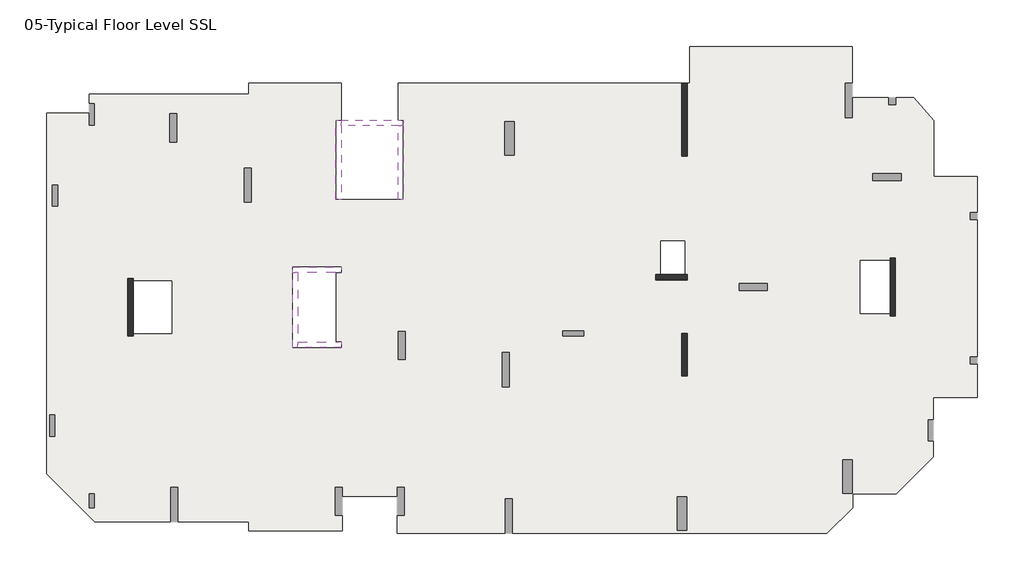
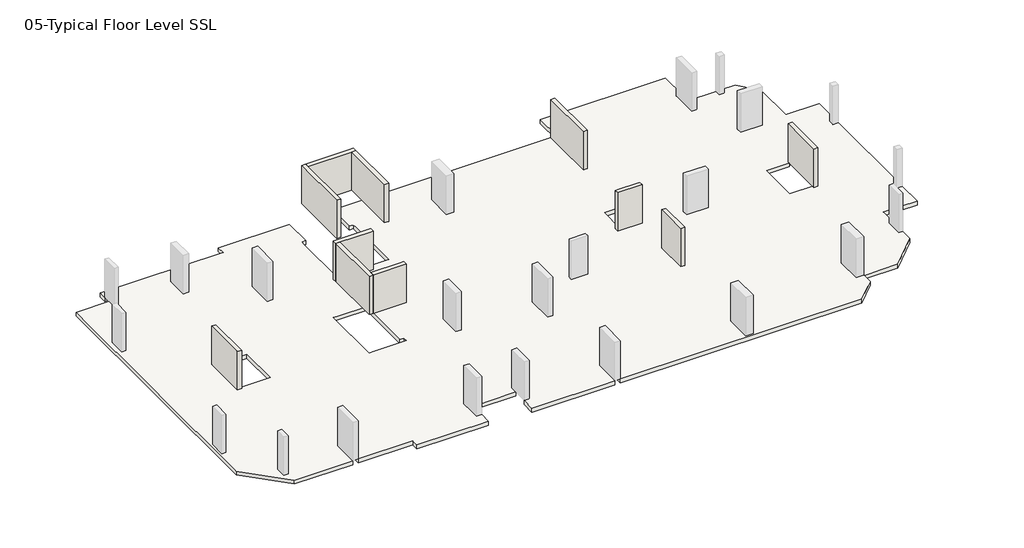
# One storey, part 1 of 2: 11 walls, 1 slab.
"""IFC4 building model written with IfcOpenShell, lengths in millimetres."""

from ifc_helpers import new_model, si_unit, origin, place, context, project, spatial, faceted_brep, element, save

model = new_model("IFC4")

# Units and contexts
model_context = context("Model", 3, world=origin())
ifc_project = project(units=[si_unit("LENGTHUNIT", "METRE", prefix="MILLI")], contexts=[model_context])

# Site, building, storey
site = spatial("IfcSite", under=ifc_project)
building = spatial("IfcBuilding", under=site)
storey = spatial("IfcBuildingStorey", under=building, Name="05-Typical Floor Level SSL", Elevation=9000.0)

# Slab
placement = place(None, origin())
element("IfcSlab", 1, ObjectType="Generic 300mm", at=placement, inside=storey, context=model_context, shape_type="Brep", body=[
    faceted_brep([(36192.0021644, 24072.000519, 8700.0), (36192.0021644, 26172.000519, 8700.0), (45446.0007483, 26172.000519, 8700.0), (45446.0007483, 24087.0, 8700.0), (45046.0007483, 24087.0, 8700.0), (45046.0007483, 22137.0, 8700.0), (45446.0007483, 22137.0, 8700.0), (45446.0007483, 23252.0000315, 8700.0), (47498.6337868, 23252.0000315, 8700.0), (47498.6337868, 22852.0, 8700.0), (47898.6337868, 22852.0, 8700.0), (47898.6337868, 23252.0000315, 8700.0), (48936.764334, 23252.0000315, 8700.0), (50076.0016214, 21956.8283806, 8700.0), (50076.0016214, 18780.0084406, 8700.0), (52549.9999998, 18780.0084406, 8700.0), (52549.9999998, 16712.0, 8700.0), (52149.9999998, 16712.0, 8700.0), (52149.9999998, 16312.0, 8700.0), (52549.9999998, 16312.0, 8700.0), (52549.9999998, 8504.0039609, 8700.0), (52149.9999998, 8504.0039609, 8700.0), (52149.9999998, 8104.0039609, 8700.0), (52549.9999998, 8104.0039609, 8700.0), (52549.9999998, 6204.0084406, 8700.0), (50046.0009271, 6204.0084406, 8700.0), (50046.0009271, 4931.9999929, 8700.0), (49746.0009271, 4931.9999929, 8700.0), (49746.0009271, 3731.9999929, 8700.0), (50046.0009271, 3731.9999929, 8700.0), (50046.0009271, 2810.5958657, 8700.0), (47943.4055804, 708.000519, 8700.0), (45456.0017287, 708.000519, 8700.0), (45456.0017287, -61.7051085, 8700.0), (43990.7023722, -1527.004465, 8700.0), (26113.9999998, -1527.004465, 8700.0), (26113.9999998, 422.995535, 8700.0), (25713.9999998, 422.995535, 8700.0), (25713.9999998, -1527.004465, 8700.0), (19569.9997488, -1527.004465, 8700.0), (19569.9997488, -512.0044652, 8700.0), (19969.9997488, -512.0044652, 8700.0), (19969.9997488, 1087.9955348, 8700.0), (19569.9997488, 1087.9955348, 8700.0), (19569.9997488, 564.000519, 8700.0), (16429.9999981, 564.000519, 8700.0), (16429.9999981, 1088.0, 8700.0), (16029.9999981, 1088.0, 8700.0), (16029.9999981, -512.0, 8700.0), (16429.9999981, -512.0, 8700.0), (16429.9999981, -1391.999481, 8700.0), (11136.0000923, -1391.999481, 8700.0), (11136.0000923, -866.9999847, 8700.0), (7082.0000416, -866.9999847, 8700.0), (7082.0000416, 1083.0000153, 8700.0), (6682.0000416, 1083.0000153, 8700.0), (6682.0000416, -866.9999847, 8700.0), (2364.4419097, -866.9999847, 8700.0), (-372.0, 1869.441925, 8700.0), (-372.0, 22380.0004589, 8700.0), (2052.0, 22380.0004589, 8700.0), (2052.0, 21708.0000656, 8700.0), (2352.0, 21708.0000656, 8700.0), (2352.0, 22908.0000656, 8700.0), (2052.0, 22908.0000656, 8700.0), (2052.0, 23472.000519, 8700.0), (11136.0000923, 23472.000519, 8700.0), (11136.0000923, 24072.000519, 8700.0), (16380.0000168, 24072.000519, 8700.0), (16380.0000168, 21972.0, 8700.0), (16079.9999997, 21972.0, 8700.0), (16079.9999997, 21672.0, 8700.0), (16079.9999997, 17468.0, 8700.0), (16379.9999997, 17468.0, 8700.0), (19619.9999997, 17468.0, 8700.0), (19919.9999997, 17468.0, 8700.0), (19919.9999997, 21672.0, 8700.0), (19919.9999997, 21972.0, 8700.0), (19619.9997365, 21972.0, 8700.0), (19619.9997365, 24072.000519, 8700.0), (35747.9999998, 24072.000519, 8700.0), (35747.9999998, 19932.0, 8700.0), (36047.9999998, 19932.0, 8700.0), (36047.9999998, 24072.000519, 8700.0), (16079.9999907, 9359.999998, 8700.0), (16079.9999907, 13320.0000002, 8700.0), (16380.0000168, 13320.0000002, 8700.0), (16380.0000168, 13620.0000002, 8700.0), (13919.9999907, 13620.0000002, 8700.0), (13619.9999907, 13620.0000002, 8700.0), (13619.9999907, 13320.0000002, 8700.0), (13619.9999907, 9359.999998, 8700.0), (13619.9999907, 9059.999998, 8700.0), (13919.9999907, 9059.999998, 8700.0), (16380.0000168, 9059.999998, 8700.0), (16380.0000168, 9359.999998, 8700.0), (257.9999999, 17088.0, 8700.0), (257.9999999, 18288.0, 8700.0), (-42.0000001, 18288.0, 8700.0), (-42.0000001, 17088.0, 8700.0), (108.001803, 4001.9999858, 8700.0), (108.001803, 5201.9999858, 8700.0), (-191.998197, 5201.9999858, 8700.0), (-191.998197, 4001.9999858, 8700.0), (30175.9999998, 9996.0000019, 8700.0), (28975.9999998, 9996.0000019, 8700.0), (28975.9999998, 9696.0000019, 8700.0), (30175.9999998, 9696.0000019, 8700.0), (7021.9999999, 20740.0000078, 8700.0), (7021.9999999, 22340.0000078, 8700.0), (6621.9999999, 22340.0000078, 8700.0), (6621.9999999, 20740.0000078, 8700.0), (48205.9993605, 18950.0, 8700.0), (46605.9993605, 18950.0, 8700.0), (46605.9993605, 18550.0, 8700.0), (48205.9993605, 18550.0, 8700.0), (20030.000009, 8355.9999979, 8700.0), (20030.000009, 9955.9999979, 8700.0), (19630.000009, 9955.9999979, 8700.0), (19630.000009, 8355.9999979, 8700.0), (11270.0000427, 17312.9999996, 8700.0), (11270.0000427, 19262.9999996, 8700.0), (10870.0000427, 19262.9999996, 8700.0), (10870.0000427, 17312.9999996, 8700.0), (40598.0014887, 12692.0079212, 8700.0), (38998.0014887, 12692.0079212, 8700.0), (38998.0014887, 12292.0079212, 8700.0), (40598.0014887, 12292.0079212, 8700.0), (25934.0000455, 6801.0001824, 8700.0), (25934.0000455, 8751.0001824, 8700.0), (25534.0000455, 8751.0001824, 8700.0), (25534.0000455, 6801.0001824, 8700.0), (36035.9999998, -1351.9992017, 8700.0), (36035.9999998, 548.0007983, 8700.0), (35485.9999998, 548.0007983, 8700.0), (35485.9999998, -1351.9992017, 8700.0), (45443.9999998, 748.0, 8700.0), (45443.9999998, 2648.0, 8700.0), (44893.9999998, 2648.0, 8700.0), (44893.9999998, 748.0, 8700.0), (26218.9999998, 20000.0, 8700.0), (26218.9999998, 21900.0, 8700.0), (25668.9999998, 21900.0, 8700.0), (25668.9999998, 20000.0, 8700.0), (2352.0, -72.0, 8700.0), (2352.0, 728.0, 8700.0), (2052.0, 728.0, 8700.0), (2052.0, -72.0, 8700.0), (4248.0000025, 12984.0000001, 8700.0), (4248.0000025, 9696.0, 8700.0), (4548.0000025, 9696.0, 8700.0), (4548.0000025, 9840.0000003, 8700.0), (6743.9999995, 9840.0000003, 8700.0), (6743.9999995, 12840.0000003, 8700.0), (4548.0000034, 12840.0000003, 8700.0), (4548.0000025, 12984.0000001, 8700.0), (34248.0015201, 12899.9999992, 8700.0), (36048.0015201, 12899.9999992, 8700.0), (36048.0015201, 13199.9999992, 8700.0), (35904.002157, 13199.9999992, 8700.0), (35904.002157, 15108.0000083, 8700.0), (34548.0015145, 15108.0000083, 8700.0), (34548.0015145, 13199.9999992, 8700.0), (34248.0015201, 13199.9999992, 8700.0), (35748.0054035, 9840.0000002, 8700.0), (35748.0054035, 7428.0000762, 8700.0), (36048.0054035, 7428.0000762, 8700.0), (36048.0054035, 9840.0000002, 8700.0), (47580.0014811, 14136.0000002, 8700.0), (47580.0014811, 13992.0079177, 8700.0), (45900.001729, 13992.0079177, 8700.0), (45900.001729, 10992.0079181, 8700.0), (47580.0014798, 10992.0079181, 8700.0), (47580.0014811, 10848.0079202, 8700.0), (47880.0014811, 10848.0079202, 8700.0), (47880.0014811, 14136.0000002, 8700.0), (36192.0021644, 26172.000519, 9000.0), (36192.0021644, 24072.000519, 9000.0), (36047.9999998, 24072.000519, 9000.0), (36047.9999998, 19932.0, 9000.0), (35747.9999998, 19932.0, 9000.0), (35747.9999998, 24072.000519, 9000.0), (19619.9997365, 24072.000519, 9000.0), (19619.9997365, 21972.0, 9000.0), (19919.9999997, 21972.0, 9000.0), (19919.9999997, 21672.0, 9000.0), (19919.9999997, 17468.0, 9000.0), (19619.9999997, 17468.0, 9000.0), (16379.9999997, 17468.0, 9000.0), (16079.9999997, 17468.0, 9000.0), (16079.9999997, 21672.0, 9000.0), (16079.9999997, 21972.0, 9000.0), (16380.0000168, 21972.0, 9000.0), (16380.0000168, 24072.000519, 9000.0), (11136.0000923, 24072.000519, 9000.0), (11136.0000923, 23472.000519, 9000.0), (2052.0, 23472.000519, 9000.0), (2052.0, 22908.0000656, 9000.0), (2352.0, 22908.0000656, 9000.0), (2352.0, 21708.0000656, 9000.0), (2052.0, 21708.0000656, 9000.0), (2052.0, 22380.0004589, 9000.0), (-372.0, 22380.0004589, 9000.0), (-372.0, 1869.441925, 9000.0), (2364.4419097, -866.9999847, 9000.0), (6682.0000416, -866.9999847, 9000.0), (6682.0000416, 1083.0000153, 9000.0), (7082.0000416, 1083.0000153, 9000.0), (7082.0000416, -866.9999847, 9000.0), (11136.0000923, -866.9999847, 9000.0), (11136.0000923, -1391.999481, 9000.0), (16429.9999981, -1391.999481, 9000.0), (16429.9999981, -512.0, 9000.0), (16029.9999981, -512.0, 9000.0), (16029.9999981, 1088.0, 9000.0), (16429.9999981, 1088.0, 9000.0), (16429.9999981, 564.000519, 9000.0), (19569.9997488, 564.000519, 9000.0), (19569.9997488, 1087.9955348, 9000.0), (19969.9997488, 1087.9955348, 9000.0), (19969.9997488, -512.0044652, 9000.0), (19569.9997488, -512.0044652, 9000.0), (19569.9997488, -1527.004465, 9000.0), (25713.9999998, -1527.004465, 9000.0), (25713.9999998, 422.995535, 9000.0), (26113.9999998, 422.995535, 9000.0), (26113.9999998, -1527.004465, 9000.0), (43990.7023722, -1527.004465, 9000.0), (45456.0017287, -61.7051085, 9000.0), (45456.0017287, 708.000519, 9000.0), (47943.4055804, 708.000519, 9000.0), (50046.0009271, 2810.5958657, 9000.0), (50046.0009271, 3731.9999929, 9000.0), (49746.0009271, 3731.9999929, 9000.0), (49746.0009271, 4931.9999929, 9000.0), (50046.0009271, 4931.9999929, 9000.0), (50046.0009271, 6204.0084406, 9000.0), (52549.9999998, 6204.0084406, 9000.0), (52549.9999998, 8104.0039609, 9000.0), (52149.9999998, 8104.0039609, 9000.0), (52149.9999998, 8504.0039609, 9000.0), (52549.9999998, 8504.0039609, 9000.0), (52549.9999998, 16312.0, 9000.0), (52149.9999998, 16312.0, 9000.0), (52149.9999998, 16712.0, 9000.0), (52549.9999998, 16712.0, 9000.0), (52549.9999998, 18780.0084406, 9000.0), (50076.0016214, 18780.0084406, 9000.0), (50076.0016214, 21956.8283806, 9000.0), (48936.764334, 23252.0000315, 9000.0), (47898.6337868, 23252.0000315, 9000.0), (47898.6337868, 22852.0, 9000.0), (47498.6337868, 22852.0, 9000.0), (47498.6337868, 23252.0000315, 9000.0), (45446.0006898, 23252.0000315, 9000.0), (45446.0007483, 22137.0, 9000.0), (45046.0007483, 22137.0, 9000.0), (45046.0007483, 24087.0, 9000.0), (45446.0007483, 24087.0, 9000.0), (45446.0007483, 26172.000519, 9000.0), (16079.9999907, 13320.0000002, 9000.0), (16079.9999907, 9359.999998, 9000.0), (16380.0000168, 9359.999998, 9000.0), (16380.0000168, 9059.999998, 9000.0), (13919.9999907, 9059.999998, 9000.0), (13619.9999907, 9059.999998, 9000.0), (13619.9999907, 9359.999998, 9000.0), (13619.9999907, 13320.0000002, 9000.0), (13619.9999907, 13620.0000002, 9000.0), (13919.9999907, 13620.0000002, 9000.0), (16380.0000168, 13620.0000002, 9000.0), (16380.0000168, 13320.0000002, 9000.0), (257.9999999, 18288.0, 9000.0), (257.9999999, 17088.0, 9000.0), (-42.0000001, 17088.0, 9000.0), (-42.0000001, 18288.0, 9000.0), (108.001803, 5201.9999858, 9000.0), (108.001803, 4001.9999858, 9000.0), (-191.998197, 4001.9999858, 9000.0), (-191.998197, 5201.9999858, 9000.0), (28975.9999998, 9996.0000019, 9000.0), (30175.9999998, 9996.0000019, 9000.0), (30175.9999998, 9696.0000019, 9000.0), (28975.9999998, 9696.0000019, 9000.0), (7021.9999999, 22340.0000078, 9000.0), (7021.9999999, 20740.0000078, 9000.0), (6621.9999999, 20740.0000078, 9000.0), (6621.9999999, 22340.0000078, 9000.0), (46605.9993605, 18950.0, 9000.0), (48205.9993605, 18950.0, 9000.0), (48205.9993605, 18550.0, 9000.0), (46605.9993605, 18550.0, 9000.0), (20030.000009, 9955.9999979, 9000.0), (20030.000009, 8355.9999979, 9000.0), (19630.000009, 8355.9999979, 9000.0), (19630.000009, 9955.9999979, 9000.0), (11270.0000427, 19262.9999996, 9000.0), (11270.0000427, 17312.9999996, 9000.0), (10870.0000427, 17312.9999996, 9000.0), (10870.0000427, 19262.9999996, 9000.0), (38998.0014887, 12692.0079212, 9000.0), (40598.0014887, 12692.0079212, 9000.0), (40598.0014887, 12292.0079212, 9000.0), (38998.0014887, 12292.0079212, 9000.0), (25934.0000455, 8751.0001824, 9000.0), (25934.0000455, 6801.0001824, 9000.0), (25534.0000455, 6801.0001824, 9000.0), (25534.0000455, 8751.0001824, 9000.0), (36035.9999998, 548.0007983, 9000.0), (36035.9999998, -1351.9992017, 9000.0), (35485.9999998, -1351.9992017, 9000.0), (35485.9999998, 548.0007983, 9000.0), (45443.9999998, 2648.0, 9000.0), (45443.9999998, 748.0, 9000.0), (44893.9999998, 748.0, 9000.0), (44893.9999998, 2648.0, 9000.0), (26218.9999998, 21900.0, 9000.0), (26218.9999998, 20000.0, 9000.0), (25668.9999998, 20000.0, 9000.0), (25668.9999998, 21900.0, 9000.0), (4248.0000025, 9696.0, 9000.0), (4248.0000025, 12984.0000001, 9000.0), (4548.0000025, 12984.0000001, 9000.0), (4548.0000025, 12840.0000003, 9000.0), (6743.9999995, 12840.0000003, 9000.0), (6743.9999995, 9840.0000003, 9000.0), (4548.0000034, 9840.0000003, 9000.0), (4548.0000025, 9696.0, 9000.0), (36048.0015201, 12899.9999992, 9000.0), (34248.0015201, 12899.9999992, 9000.0), (34248.0015201, 13199.9999992, 9000.0), (34548.0015145, 13199.9999992, 9000.0), (34548.0015145, 15108.0000083, 9000.0), (35904.002157, 15108.0000083, 9000.0), (35904.002157, 13199.9999992, 9000.0), (36048.0015201, 13199.9999992, 9000.0), (35748.0054035, 7428.0000762, 9000.0), (35748.0054035, 9840.0000002, 9000.0), (36048.0054035, 9840.0000002, 9000.0), (36048.0054035, 7428.0000762, 9000.0), (47880.0014811, 14136.0000002, 9000.0), (47880.0014811, 10848.0079202, 9000.0), (47580.0014811, 10848.0079202, 9000.0), (47580.0014811, 10992.0079181, 9000.0), (45900.001729, 10992.0079181, 9000.0), (45900.001729, 13992.0079177, 9000.0), (47580.0014798, 13992.0079177, 9000.0), (47580.0014811, 14136.0000002, 9000.0), (2352.0, 728.0, 9000.0), (2352.0, -72.0, 9000.0), (2052.0, -72.0, 9000.0), (2052.0, 728.0, 9000.0)], [[[0, 1, 2, 3, 4, 5, 6, 7, 8, 9, 10, 11, 12, 13, 14, 15, 16, 17, 18, 19, 20, 21, 22, 23, 24, 25, 26, 27, 28, 29, 30, 31, 32, 33, 34, 35, 36, 37, 38, 39, 40, 41, 42, 43, 44, 45, 46, 47, 48, 49, 50, 51, 52, 53, 54, 55, 56, 57, 58, 59, 60, 61, 62, 63, 64, 65, 66, 67, 68, 69, 70, 71, 72, 73, 74, 75, 76, 77, 78, 79, 80, 81, 82, 83], [84, 85, 86, 87, 88, 89, 90, 91, 92, 93, 94, 95], [96, 97, 98, 99], [100, 101, 102, 103], [104, 105, 106, 107], [108, 109, 110, 111], [112, 113, 114, 115], [116, 117, 118, 119], [120, 121, 122, 123], [124, 125, 126, 127], [128, 129, 130, 131], [132, 133, 134, 135], [136, 137, 138, 139], [140, 141, 142, 143], [144, 145, 146, 147], [148, 149, 150, 151, 152, 153, 154, 155], [156, 157, 158, 159, 160, 161, 162, 163], [164, 165, 166, 167], [168, 169, 170, 171, 172, 173, 174, 175]], [[176, 177, 178, 179, 180, 181, 182, 183, 184, 185, 186, 187, 188, 189, 190, 191, 192, 193, 194, 195, 196, 197, 198, 199, 200, 201, 202, 203, 204, 205, 206, 207, 208, 209, 210, 211, 212, 213, 214, 215, 216, 217, 218, 219, 220, 221, 222, 223, 224, 225, 226, 227, 228, 229, 230, 231, 232, 233, 234, 235, 236, 237, 238, 239, 240, 241, 242, 243, 244, 245, 246, 247, 248, 249, 250, 251, 252, 253, 254, 255, 256, 257, 258, 259], [260, 261, 262, 263, 264, 265, 266, 267, 268, 269, 270, 271], [272, 273, 274, 275], [276, 277, 278, 279], [280, 281, 282, 283], [284, 285, 286, 287], [288, 289, 290, 291], [292, 293, 294, 295], [296, 297, 298, 299], [300, 301, 302, 303], [304, 305, 306, 307], [308, 309, 310, 311], [312, 313, 314, 315], [316, 317, 318, 319], [320, 321, 322, 323, 324, 325, 326, 327], [328, 329, 330, 331, 332, 333, 334, 335], [336, 337, 338, 339], [340, 341, 342, 343, 344, 345, 346, 347], [348, 349, 350, 351]], [[68, 193, 192, 69]], [[182, 79, 78, 183]], [[79, 182, 181, 80]], [[177, 0, 83, 178]], [[1, 0, 177, 176]], [[2, 1, 176, 259]], [[3, 2, 259, 258]], [[249, 12, 11, 250]], [[7, 254, 253, 8]], [[13, 12, 249, 248]], [[14, 13, 248, 247]], [[15, 14, 247, 246]], [[15, 246, 245, 16]], [[237, 24, 23, 238]], [[19, 242, 241, 20]], [[25, 24, 237, 236]], [[25, 236, 235, 26]], [[30, 29, 232, 231]], [[32, 31, 230, 229]], [[33, 32, 229, 228]], [[34, 33, 228, 227]], [[34, 227, 226, 35]], [[222, 39, 38, 223]], [[39, 222, 221, 40]], [[45, 44, 217, 216]], [[211, 50, 49, 212]], [[51, 50, 211, 210]], [[52, 51, 210, 209]], [[52, 209, 208, 53]], [[204, 57, 56, 205]], [[58, 57, 204, 203]], [[59, 58, 203, 202]], [[60, 59, 202, 201]], [[196, 65, 64, 197]], [[66, 65, 196, 195]], [[67, 66, 195, 194]], [[68, 67, 194, 193]], [[85, 84, 261, 260]], [[62, 199, 198, 63]], [[199, 62, 61, 200]], [[200, 61, 60, 201]], [[63, 198, 197, 64]], [[96, 273, 272, 97]], [[273, 96, 99, 274]], [[274, 99, 98, 275]], [[275, 98, 97, 272]], [[100, 277, 276, 101]], [[277, 100, 103, 278]], [[278, 103, 102, 279]], [[279, 102, 101, 276]], [[28, 233, 232, 29]], [[233, 28, 27, 234]], [[234, 27, 26, 235]], [[104, 281, 280, 105]], [[281, 104, 107, 282]], [[282, 107, 106, 283]], [[283, 106, 105, 280]], [[108, 285, 284, 109]], [[285, 108, 111, 286]], [[286, 111, 110, 287]], [[287, 110, 109, 284]], [[41, 220, 219, 42]], [[220, 41, 40, 221]], [[43, 218, 217, 44]], [[218, 43, 42, 219]], [[112, 289, 288, 113]], [[289, 112, 115, 290]], [[290, 115, 114, 291]], [[291, 114, 113, 288]], [[116, 293, 292, 117]], [[293, 116, 119, 294]], [[294, 119, 118, 295]], [[295, 118, 117, 292]], [[215, 46, 45, 216]], [[48, 213, 212, 49]], [[213, 48, 47, 214]], [[214, 47, 46, 215]], [[120, 297, 296, 121]], [[297, 120, 123, 298]], [[298, 123, 122, 299]], [[299, 122, 121, 296]], [[207, 54, 53, 208]], [[55, 206, 205, 56]], [[206, 55, 54, 207]], [[225, 36, 35, 226]], [[37, 224, 223, 38]], [[224, 37, 36, 225]], [[6, 255, 254, 7]], [[255, 6, 5, 256]], [[256, 5, 4, 257]], [[257, 4, 3, 258]], [[124, 301, 300, 125]], [[301, 124, 127, 302]], [[302, 127, 126, 303]], [[303, 126, 125, 300]], [[128, 305, 304, 129]], [[305, 128, 131, 306]], [[306, 131, 130, 307]], [[307, 130, 129, 304]], [[132, 309, 308, 133]], [[309, 132, 135, 310]], [[310, 135, 134, 311]], [[311, 134, 133, 308]], [[136, 313, 312, 137]], [[313, 136, 139, 314]], [[314, 139, 138, 315]], [[315, 138, 137, 312]], [[140, 317, 316, 141]], [[317, 140, 143, 318]], [[318, 143, 142, 319]], [[319, 142, 141, 316]], [[144, 349, 348, 145]], [[349, 144, 147, 350]], [[146, 351, 350, 147]], [[145, 348, 351, 146]], [[70, 191, 190, 189, 72, 71]], [[191, 70, 69, 192]], [[77, 184, 183, 78]], [[184, 77, 76, 75, 186, 185]], [[271, 86, 85, 260]], [[87, 270, 269, 268, 89, 88]], [[86, 271, 270, 87]], [[89, 268, 267, 266, 265, 92, 91, 90]], [[92, 265, 264, 263, 94, 93]], [[95, 262, 261, 84]], [[262, 95, 94, 263]], [[322, 155, 154, 323]], [[150, 327, 326, 151]], [[148, 321, 320, 149]], [[155, 322, 321, 148]], [[327, 150, 149, 320]], [[156, 329, 328, 157]], [[158, 335, 334, 159]], [[330, 163, 162, 331]], [[157, 328, 335, 158]], [[329, 156, 163, 330]], [[164, 337, 336, 165]], [[166, 339, 338, 167]], [[165, 336, 339, 166]], [[337, 164, 167, 338]], [[342, 173, 172, 343]], [[168, 347, 346, 169]], [[174, 341, 340, 175]], [[173, 342, 341, 174]], [[347, 168, 175, 340]], [[82, 179, 178, 83]], [[180, 81, 80, 181]], [[179, 82, 81, 180]], [[72, 189, 188, 187, 186, 75, 74, 73]], [[325, 152, 151, 326]], [[152, 325, 324, 153]], [[153, 324, 323, 154]], [[345, 170, 169, 346]], [[170, 345, 344, 171]], [[171, 344, 343, 172]], [[160, 333, 332, 161]], [[161, 332, 331, 162]], [[333, 160, 159, 334]], [[31, 30, 231, 230]], [[18, 243, 242, 19]], [[243, 18, 17, 244]], [[244, 17, 16, 245]], [[10, 251, 250, 11]], [[251, 10, 9, 252]], [[252, 9, 8, 253]], [[22, 239, 238, 23]], [[239, 22, 21, 240]], [[240, 21, 20, 241]]]),
])

# Walls
element("IfcWall", 2, ObjectType="Shear Walls 300mm", at=placement, inside=storey, context=model_context, shape_type="Brep", body=[
    faceted_brep([(4548.0000025, 9696.0, 9000.0), (4548.0000025, 12984.0000001, 9000.0), (4548.0000025, 12984.0000001, 11700.0), (4548.0000025, 12984.0000001, 12000.0), (4548.0000025, 12840.0000003, 12000.0), (4548.0000025, 9840.0000003, 12000.0), (4548.0000025, 9696.0, 12000.0), (4548.0000025, 9696.0, 11700.0), (4248.0000025, 9696.0, 9000.0), (4248.0000025, 9696.0, 11700.0), (4248.0000025, 9696.0, 12000.0), (4248.0000025, 12984.0000001, 12000.0), (4248.0000025, 12984.0000001, 11700.0), (4248.0000025, 12984.0000001, 9000.0)], [[[0, 1, 2, 3, 4, 5, 6, 7]], [[8, 9, 10, 11, 12, 13]], [[1, 0, 8, 13]], [[3, 2, 1, 13, 12, 11]], [[6, 5, 4, 3, 11, 10]], [[0, 7, 6, 10, 9, 8]]]),
])
element("IfcWall", 3, ObjectType="Shear Walls 300mm", at=placement, inside=storey, context=model_context, shape_type="Brep", body=[
    faceted_brep([(34248.0015201, 12899.9999992, 9000.0), (36048.0015201, 12899.9999992, 9000.0), (36048.0015201, 12899.9999992, 11700.0), (36048.0015201, 12899.9999992, 12000.0), (34248.0015201, 12899.9999992, 12000.0), (34248.0015201, 12899.9999992, 11700.0), (34248.0015201, 13199.9999992, 9000.0), (34248.0015201, 13199.9999992, 11700.0), (34248.0015201, 13199.9999992, 12000.0), (34548.0015145, 13199.9999992, 12000.0), (35904.002157, 13199.9999992, 12000.0), (36048.0015201, 13199.9999992, 12000.0), (36048.0015201, 13199.9999992, 11700.0), (36048.0015201, 13199.9999992, 9000.0)], [[[0, 1, 2, 3, 4, 5]], [[6, 7, 8, 9, 10, 11, 12, 13]], [[1, 0, 6, 13]], [[3, 2, 1, 13, 12, 11]], [[4, 3, 11, 10, 9, 8]], [[0, 5, 4, 8, 7, 6]]]),
])
element("IfcWall", 4, ObjectType="Shear Walls 300mm", at=placement, inside=storey, context=model_context, shape_type="Brep", body=[
    faceted_brep([(35748.0054035, 9840.0000002, 9000.0), (35748.0054035, 7428.0000762, 9000.0), (35748.0054035, 7428.0000762, 11700.0), (35748.0054035, 7428.0000762, 12000.0), (35748.0054035, 9840.0000002, 12000.0), (35748.0054035, 9840.0000002, 11700.0), (36048.0054035, 9840.0000002, 9000.0), (36048.0054035, 9840.0000002, 11700.0), (36048.0054035, 9840.0000002, 12000.0), (36048.0054035, 7428.0000762, 12000.0), (36048.0054035, 7428.0000762, 11700.0), (36048.0054035, 7428.0000762, 9000.0)], [[[0, 1, 2, 3, 4, 5]], [[6, 7, 8, 9, 10, 11]], [[1, 0, 6, 11]], [[3, 2, 1, 11, 10, 9]], [[4, 3, 9, 8]], [[0, 5, 4, 8, 7, 6]]]),
])
element("IfcWall", 5, ObjectType="Shear Walls 300mm", at=placement, inside=storey, context=model_context, shape_type="Brep", body=[
    faceted_brep([(47580.0014811, 14136.0000002, 9000.0), (47580.0014811, 10848.0079202, 9000.0), (47580.0014811, 10848.0079202, 11700.0), (47580.0014811, 10848.0079202, 12000.0), (47580.0014811, 10992.0079181, 12000.0), (47580.0014811, 13992.0079177, 12000.0), (47580.0014811, 14136.0000002, 12000.0), (47580.0014811, 14136.0000002, 11700.0), (47880.0014811, 14136.0000002, 9000.0), (47880.0014811, 14136.0000002, 11700.0), (47880.0014811, 14136.0000002, 12000.0), (47880.0014811, 10848.0079202, 12000.0), (47880.0014811, 10848.0079202, 11700.0), (47880.0014811, 10848.0079202, 9000.0)], [[[0, 1, 2, 3, 4, 5, 6, 7]], [[8, 9, 10, 11, 12, 13]], [[1, 0, 8, 13]], [[3, 2, 1, 13, 12, 11]], [[6, 5, 4, 3, 11, 10]], [[0, 7, 6, 10, 9, 8]]]),
])
element("IfcWall", 6, ObjectType="Shear Walls 300mm", at=placement, inside=storey, context=model_context, shape_type="Brep", body=[
    faceted_brep([(36047.9999998, 19932.0, 9000.0), (36047.9999998, 24072.0078999, 9000.0), (36047.9999998, 24072.0078999, 12000.0), (36047.9999998, 19932.0, 12000.0), (36047.9999998, 19932.0, 11700.0), (35747.9999998, 19932.0, 9000.0), (35747.9999998, 19932.0, 11700.0), (35747.9999998, 19932.0, 12000.0), (35747.9999998, 24072.0078999, 12000.0), (35747.9999998, 24072.0078999, 9000.0)], [[[0, 1, 2, 3, 4]], [[5, 6, 7, 8, 9]], [[1, 0, 5, 9]], [[2, 1, 9, 8]], [[3, 2, 8, 7]], [[0, 4, 3, 7, 6, 5]]]),
])
element("IfcWall", 7, ObjectType="Shear Walls 300mm", at=placement, inside=storey, context=model_context, shape_type="Brep", body=[
    faceted_brep([(16379.9999997, 21972.0, 15000.0), (16379.9999997, 21672.0, 15000.0), (16379.9999997, 17468.0, 15000.0), (16379.9999997, 17468.0, 12000.0), (16379.9999997, 21672.0, 12000.0), (16379.9999997, 21972.0, 12000.0), (16079.9999997, 17468.0, 15000.0), (16079.9999997, 21972.0, 15000.0), (16079.9999997, 21972.0, 14700.0), (16079.9999997, 21972.0, 12000.0), (16079.9999997, 17468.0, 12000.0), (16079.9999997, 17468.0, 14700.0)], [[[0, 1, 2, 3, 4, 5]], [[6, 7, 8, 9, 10, 11]], [[2, 1, 0, 7, 6]], [[2, 6, 11, 10, 3]], [[3, 10, 9, 5, 4]], [[0, 5, 9, 8, 7]]]),
])
element("IfcWall", 8, ObjectType="Shear Walls 300mm", at=placement, inside=storey, context=model_context, shape_type="Brep", body=[
    faceted_brep([(16379.9999997, 21972.0, 15000.0), (19619.9997365, 21972.0, 15000.0), (19919.9999997, 21972.0, 15000.0), (19919.9999997, 21972.0, 14700.0), (19919.9999997, 21972.0, 12000.0), (16379.9999997, 21972.0, 12000.0), (19919.9999997, 21672.0, 15000.0), (19619.9999997, 21672.0, 15000.0), (16379.9999997, 21672.0, 15000.0), (16379.9999997, 21672.0, 12000.0), (19619.9999997, 21672.0, 12000.0), (19919.9999997, 21672.0, 12000.0)], [[[0, 1, 2, 3, 4, 5]], [[6, 7, 8, 9, 10, 11]], [[2, 1, 0, 8, 7, 6]], [[8, 0, 5, 9]], [[9, 5, 4, 11, 10]], [[4, 3, 2, 6, 11]]]),
])
element("IfcWall", 9, ObjectType="Shear Walls 300mm", at=placement, inside=storey, context=model_context, shape_type="Brep", body=[
    faceted_brep([(19919.9999997, 21672.0, 15000.0), (19919.9999997, 17468.0, 15000.0), (19919.9999997, 17468.0, 14700.0), (19919.9999997, 17468.0, 12000.0), (19919.9999997, 21672.0, 12000.0), (19619.9999997, 17468.0, 15000.0), (19619.9999997, 21672.0, 15000.0), (19619.9999997, 21672.0, 12000.0), (19619.9999997, 17468.0, 12000.0)], [[[0, 1, 2, 3, 4]], [[5, 6, 7, 8]], [[1, 0, 6, 5]], [[1, 5, 8, 3, 2]], [[6, 0, 4, 7]], [[4, 3, 8, 7]]]),
])
element("IfcWall", 10, ObjectType="Shear Walls 300mm", at=placement, inside=storey, context=model_context, shape_type="Brep", body=[
    faceted_brep([(16380.0000168, 13320.0000002, 15000.0), (16079.9999907, 13320.0000002, 15000.0), (13919.9999907, 13320.0000002, 15000.0), (13619.9999907, 13320.0000002, 15000.0), (13619.9999907, 13320.0000002, 12000.0), (13919.9999907, 13320.0000002, 12000.0), (16380.0000168, 13320.0000002, 12000.0), (16380.0000168, 13320.0000002, 14700.0), (13619.9999907, 13620.0000002, 15000.0), (16380.0000168, 13620.0000002, 15000.0), (16380.0000168, 13620.0000002, 14700.0), (16380.0000168, 13620.0000002, 12000.0), (13619.9999907, 13620.0000002, 12000.0), (13619.9999907, 13620.0000002, 14700.0)], [[[0, 1, 2, 3, 4, 5, 6, 7]], [[8, 9, 10, 11, 12, 13]], [[9, 0, 7, 6, 11, 10]], [[3, 2, 1, 0, 9, 8]], [[11, 6, 5, 4, 12]], [[4, 3, 8, 13, 12]]]),
])
element("IfcWall", 11, ObjectType="Shear Walls 300mm", at=placement, inside=storey, context=model_context, shape_type="Brep", body=[
    faceted_brep([(13919.9999907, 13320.0000002, 15000.0), (13919.9999907, 9359.999998, 15000.0), (13919.9999907, 9059.999998, 15000.0), (13919.9999907, 9059.999998, 12000.0), (13919.9999907, 9359.999998, 12000.0), (13919.9999907, 13320.0000002, 12000.0), (13619.9999907, 9059.999998, 15000.0), (13619.9999907, 13320.0000002, 15000.0), (13619.9999907, 13320.0000002, 12000.0), (13619.9999907, 9059.999998, 12000.0), (13619.9999907, 9059.999998, 14700.0)], [[[0, 1, 2, 3, 4, 5]], [[6, 7, 8, 9, 10]], [[2, 1, 0, 7, 6]], [[7, 0, 5, 8]], [[8, 5, 4, 3, 9]], [[3, 2, 6, 10, 9]]]),
])
element("IfcWall", 12, ObjectType="Shear Walls 300mm", at=placement, inside=storey, context=model_context, shape_type="Brep", body=[
    faceted_brep([(13919.9999907, 9359.999998, 15000.0), (16079.9999907, 9359.999998, 15000.0), (16380.0000168, 9359.999998, 15000.0), (16380.0000168, 9359.999998, 14700.0), (16380.0000168, 9359.999998, 12000.0), (13919.9999907, 9359.999998, 12000.0), (16380.0000168, 9059.999998, 15000.0), (13919.9999907, 9059.999998, 15000.0), (13919.9999907, 9059.999998, 12000.0), (16380.0000168, 9059.999998, 12000.0), (16380.0000168, 9059.999998, 14700.0)], [[[0, 1, 2, 3, 4, 5]], [[6, 7, 8, 9, 10]], [[2, 1, 0, 7, 6]], [[2, 6, 10, 9, 4, 3]], [[7, 0, 5, 8]], [[5, 4, 9, 8]]]),
])

save(model, "model.ifc")

# Revit data of these elements
# Type "Generic 300mm"
#   Function = 0
#   Layers, outside or top first: 300 mm "Concrete-RC" (function 1)
# Type "Shear Walls 300mm"
#   Layers, outside or top first: 300 mm "Concrete-RC" (function 1)
# Element 1 (IfcSlab, "Generic 300mm")
#   Height Offset From Level = 0 mm
#   built-in parameter 1001954 = 1
#   Phase Created = New Construction
#   Materials on its faces: "Concrete-RC"
# Elements 2, 3, 4, 5, 6 (IfcWall, "Shear Walls 300mm")
#   Top Offset = 0 mm
#   Base Offset = 0 mm
#   wall height = 3000 mm
#   Phase Created = New Construction
#   Base Constraint = 05-Typical Floor Level SSL
#   Top Constraint = 06-Typical Floor Level SSL
#   Materials on its faces: "Concrete-RC"
# Elements 7, 8, 9, 10, 11, 12 (IfcWall, "Shear Walls 300mm")
#   Top Offset = 0 mm
#   Base Offset = 0 mm
#   wall height = 6000 mm
#   Phase Created = New Construction
#   Base Constraint = 05-Typical Floor Level SSL
#   Top Constraint = 07-Typical Floor Level SSL
#   Materials on its faces: "Concrete-RC"
# Materials
#   "Concrete-RC": class "Concrete", colour RGB 128 128 128, transparency 0, Description = "High strength concrete", Cost = 0
